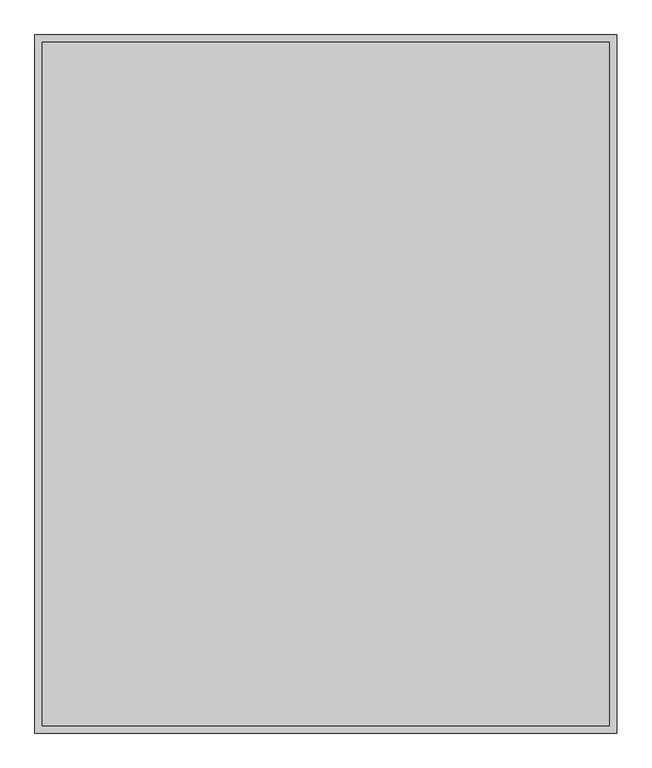
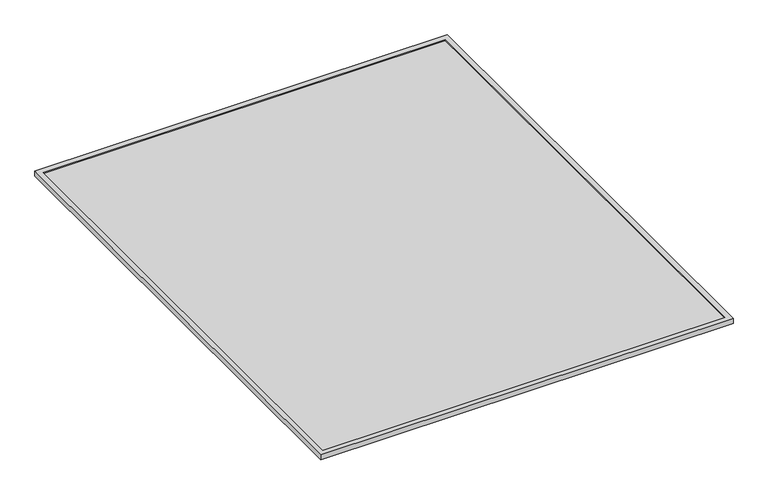
"""IFC4 building model written with IfcOpenShell, lengths in millimetres: proxy geometry, Bradley-Washroom_Accessories-Mirrors-780_Custom : Bradley-Washroom_Accessories-Mirrors-780_Custom."""

from ifc_helpers import new_model, si_unit, frame, origin, place, context, project, spatial, polyline, outline, extrude, faceted_brep, source, transform, mapped, element, save


def specialty_equipment_f3c20ec9(model_context):
    return source(origin(), model_context, "Body", "SolidModel", [
        extrude(outline(polyline([(742.95, 895.35), (742.95, -895.35), (-742.95, -895.35), (-742.95, 895.35), (742.95, 895.35)])), frame((0.0, 0.0, 9.525), z_axis=(0.0, 0.0, 1.0), x_axis=(1.0, 0.0, 0.0)), (0.0, 0.0, 1.0), 4.7625),
        faceted_brep([(762.0, 914.4, 19.05), (-762.0, 914.4, 19.05), (-762.0, -914.4, 19.05), (762.0, -914.4, 19.05), (-742.95, 895.35, 19.05), (742.95, 895.35, 19.05), (742.95, -895.35, 19.05), (-742.95, -895.35, 19.05), (762.0, 914.4, 0.0), (762.0, -914.4, 0.0), (-762.0, -914.4, 0.0), (-762.0, 914.4, 0.0), (742.95, 895.35, 9.525), (-742.95, 895.35, 9.525), (-742.95, -895.35, 9.525), (742.95, -895.35, 9.525)], [[[0, 1, 2, 3], [4, 5, 6, 7]], [[8, 9, 10, 11]], [[1, 0, 8, 11]], [[2, 1, 11, 10]], [[3, 2, 10, 9]], [[0, 3, 9, 8]], [[12, 13, 14, 15]], [[13, 12, 5, 4]], [[14, 13, 4, 7]], [[15, 14, 7, 6]], [[12, 15, 6, 5]]]),
    ])


if __name__ == "__main__":
    model = new_model("IFC4")
    model_context = context("Model", 3, world=origin())
    ifc_project = project(units=[si_unit("LENGTHUNIT", "METRE", prefix="MILLI")], contexts=[model_context])
    site = spatial("IfcSite", under=ifc_project)
    building = spatial("IfcBuilding", under=site)
    placement = place(None, origin())
    specialty_equipment_shape = specialty_equipment_f3c20ec9(model_context)
    element("IfcBuildingElementProxy", 1, Name="Bradley-Washroom_Accessories-Mirrors-780_Custom : Bradley-Washroom_Accessories-Mirrors-780_Custom", ObjectType="Bradley-Washroom_Accessories-Mirrors-780_Custom : Bradley-Washroom_Accessories-Mirrors-780_Custom", at=placement, inside=building, context=model_context, shape_type="MappedRepresentation", body=[
        mapped(specialty_equipment_shape, transform((0.0, 0.0, 0.0), x_axis=(1.0, 0.0, 0.0), y_axis=(0.0, 1.0, 0.0), z_axis=(0.0, 0.0, 1.0))),
    ])
    save(model, "model.ifc")

# Revit data of these elements
# Type "Bradley-Washroom_Accessories-Mirrors-780_Custom : Bradley-Washroom_Accessories-Mirrors-780_Custom"
#   Keynote = "M08831300.01"
#   Warranty Information = "Complete unit, excepting mirrors warranted for one year.\r\n Stainless steel mirror frames for fifteen years.\r\n Plate glass mirrors for fifteen years.\r\n This warranty does not cover installation or any other labor charges and does not apply to any units,\r\n which have been damaged by accident, abuse, improper installation, improper maintenance, or altered in any way."
#   Version = "1.0"
#   URL = "http://www.bradleycorp.com/"
#   Type Comments = "ERROR - If you are able to see this message you haven't loaded this  family correctly."
#   OmniClass Title = "Mirrors"
#   OmniClass Code = "23.40.95.17.17"
#   Modeling Code = ""
#   Model = "ERROR - If you are able to see this message you haven't loaded this  family correctly."
#   MasterFormat Title = "Commercial Toilet Accessories"
#   MasterFormat Number = "10 28 13. 13"
#   Manufacturer = "Bradley Corporation"
#   Industry Standards = "ASTM C 1036"
#   Fire Rating = "n/a"
#   Dimensional Limits [instance default] = "Either Width or Hight must be over 25\""
#   Description = "ERROR - If you are able to see this message you haven't loaded this  family correctly."
#   Copyright = "This Model Data is Property of Bradley Corporation"
#   Buy American Act = "Yes"
#   Assembly Code = "C1030900"
#   ADA Compliant = "Yes"
#   Width [instance default] = 1' - 6"
#   Total Width [instance default] = 1' - 6"
#   Total Height [instance default] = 3' - 0"
#   Height [instance default] = 3' - 0"
#   Depth [instance default] = 0' - 0 3/4"
#   Default Elevation = 3' - 4"
#   Reflective Material = Glass - Bradley Corp - BradEX - Polished Float Mirror
#   Frame Material = Bradley Corp Stainless Steel - Satin
# Element 1 (IfcBuildingElementProxy, "Bradley-Washroom_Accessories-Mirrors-780_Custom : Bradley-Washroom_Accessories-Mirrors-780_Custom")
#   Width = 5' - 0"
#   Total Width = 5' - 0"
#   Total Height = 6' - 0"
#   Height = 6' - 0"
#   Materials on its faces: "Bradley Corp Stainless Steel - Satin", "Glass - Bradley Corp - BradEX - Polished Float Mirror"
# Materials
#   "Glass - Bradley Corp - BradEX - Polished Float Mirror": class "Glass", colour RGB 221 230 232, transparency 0, Manufacturer = "Bradley Corporation", URL = "www.bradleycorp.com", Description = "Stainless Steel - Satin Finish", Cost = 0
#   "Bradley Corp Stainless Steel - Satin": class "Metal", colour RGB 189 187 185, transparency 0, Manufacturer = "Bradley Corporation", URL = "www.bradleycorp.com", Description = "Stainless Steel - Satin Finish", Cost = 0
